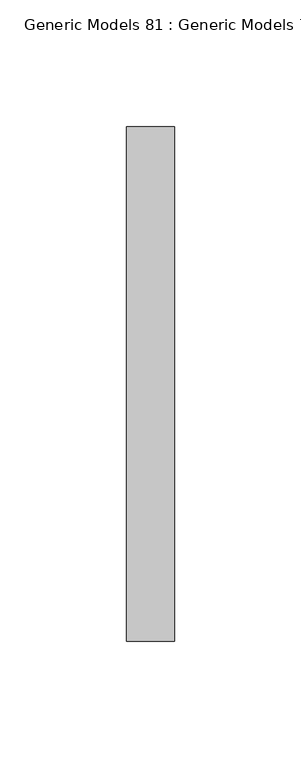
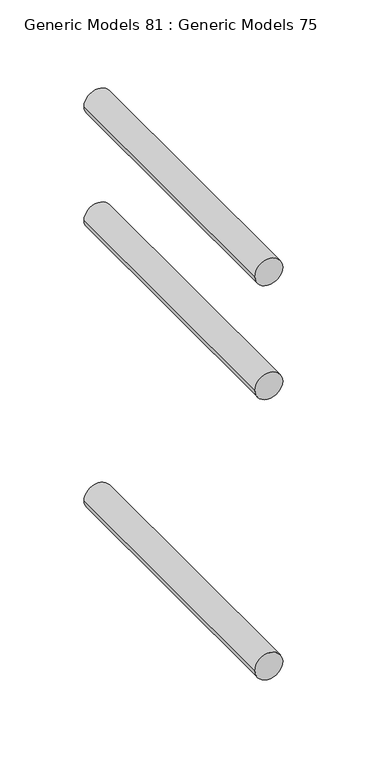
"""IFC4 building model written with IfcOpenShell, lengths in millimetres: proxy geometry, Generic Models 81 : Generic Models 75."""

import ifcopenshell
import ifcopenshell.guid

model = None  # the IFC model being written
_history = None  # IfcOwnerHistory: only IFC2X3 demands one
_inside = {}  # id of a spatial element -> (the spatial element, [elements in it])
_under = {}  # id of a project, library or spatial element -> (it, [spatial elements below it])
_declared = {}  # id of a project -> (the project, [libraries it declares])
_typed = {}  # id of a type object -> (the type object, [elements of that type])
_made_of = {}  # id of a material, layer set ... -> (it, [elements and type objects made of it])


def new_model(schema):
    """Start an empty IFC model of exactly this schema.

    Asked for "IFC4X3", IfcOpenShell would pick the latest addendum, in which some entities
    have other attributes; the version numbers below select the first issue.
    IFC2X3 requires an IfcOwnerHistory on every rooted entity: one is made here for all.
    """
    global model, _history
    if schema == "IFC4X3":
        model = ifcopenshell.file(schema_version=(4, 3, 0, 0))
    else:
        model = ifcopenshell.file(schema=schema)
    _inside.clear()
    _under.clear()
    _declared.clear()
    _typed.clear()
    _made_of.clear()
    _history = None
    if model.schema == "IFC2X3":
        org = make("IfcOrganization", Name="unknown")
        user = make(
            "IfcPersonAndOrganization",
            ThePerson=make("IfcPerson", FamilyName="unknown"),
            TheOrganization=org,
        )
        app = make(
            "IfcApplication",
            ApplicationDeveloper=org,
            Version="unknown",
            ApplicationFullName="unknown",
            ApplicationIdentifier="unknown",
        )
        _history = make(
            "IfcOwnerHistory",
            OwningUser=user,
            OwningApplication=app,
            ChangeAction="ADDED",
            CreationDate=0,
        )
    return model


def make(cls, **values):
    """One entity of the class cls with the attributes given. An attribute that is None is left unset."""
    return model.create_entity(
        cls, **{name: value for name, value in values.items() if value is not None}
    )


def rooted(cls, **values):
    """An entity with a GlobalId (a new one), such as an element, a storey or a relation."""
    return make(cls, GlobalId=ifcopenshell.guid.new(), OwnerHistory=_history, **values)


def si_unit(unit_type, name, prefix=None):
    """IfcSIUnit, for example si_unit("LENGTHUNIT", "METRE", prefix="MILLI")."""
    return make("IfcSIUnit", UnitType=unit_type, Prefix=prefix, Name=name)


def assignment(units):
    """IfcUnitAssignment: the units of a project."""
    return None if units is None else make("IfcUnitAssignment", Units=units)


def point(xyz):
    """IfcCartesianPoint."""
    return None if xyz is None else make("IfcCartesianPoint", Coordinates=xyz)


def direction(xyz):
    """IfcDirection."""
    return None if xyz is None else make("IfcDirection", DirectionRatios=xyz)


def frame(location, z_axis=None, x_axis=None):
    """IfcAxis2Placement3D, a coordinate frame: its origin and axes. An axis left out is left unset."""
    return make(
        "IfcAxis2Placement3D",
        Location=point(location),
        Axis=direction(z_axis),
        RefDirection=direction(x_axis),
    )


def frame_2d(location, x_axis=None):
    """IfcAxis2Placement2D, a coordinate frame in the plane: its origin and x axis."""
    return make(
        "IfcAxis2Placement2D", Location=point(location), RefDirection=direction(x_axis)
    )


def origin():
    """The frame at (0, 0, 0) with its axes left unset."""
    return frame((0.0, 0.0, 0.0))


def place(relative_to, where):
    """IfcLocalPlacement: puts the frame where relative to a parent placement (None: the world)."""
    return make(
        "IfcLocalPlacement", PlacementRelTo=relative_to, RelativePlacement=where
    )


def context(
    kind, dimensions, precision=None, world=None, true_north=None, identifier=None
):
    """IfcGeometricRepresentationContext, for example the 3D "Model" context."""
    return make(
        "IfcGeometricRepresentationContext",
        ContextIdentifier=identifier,
        ContextType=kind,
        CoordinateSpaceDimension=dimensions,
        Precision=precision,
        WorldCoordinateSystem=world,
        TrueNorth=true_north,
    )


def project(units=None, contexts=None):
    """IfcProject with its units and contexts."""
    return rooted(
        "IfcProject",
        Name="project",
        RepresentationContexts=contexts,
        UnitsInContext=assignment(units),
    )


def spatial(cls, under=None, at=None, **own):
    """A site, building, storey or space (cls), placed at a placement, below another one or the project."""
    s = rooted(cls, ObjectPlacement=at, **own)
    if under is not None:
        _under.setdefault(under.id(), (under, []))[1].append(s)
    return s


def circle_curve(where, radius):
    """IfcCircle in the frame where."""
    return make("IfcCircle", Position=where, Radius=radius)


def trimmed(basis, trim1, trim2, sense, master):
    """IfcTrimmedCurve: the piece of a basis curve between two trims."""
    return make(
        "IfcTrimmedCurve",
        BasisCurve=basis,
        Trim1=trim1,
        Trim2=trim2,
        SenseAgreement=sense,
        MasterRepresentation=master,
    )


def segment(curve, same_sense, transition):
    """IfcCompositeCurveSegment."""
    return make(
        "IfcCompositeCurveSegment",
        Transition=transition,
        SameSense=same_sense,
        ParentCurve=curve,
    )


def composite_curve(segments, self_intersect=None):
    """IfcCompositeCurve: segments joined end to end."""
    return make("IfcCompositeCurve", Segments=segments, SelfIntersect=self_intersect)


def outline(outer, holes=None, kind="AREA"):
    """IfcArbitraryClosedProfileDef: a profile drawn as a closed curve; with holes, ...WithVoids."""
    if holes is None:
        return make("IfcArbitraryClosedProfileDef", ProfileType=kind, OuterCurve=outer)
    return make(
        "IfcArbitraryProfileDefWithVoids",
        ProfileType=kind,
        OuterCurve=outer,
        InnerCurves=holes,
    )


def extrude(swept, where, along, depth):
    """IfcExtrudedAreaSolid: the profile swept, set in the frame where, extruded along a direction by depth."""
    return make(
        "IfcExtrudedAreaSolid",
        SweptArea=swept,
        Position=where,
        ExtrudedDirection=direction(along),
        Depth=depth,
    )


def shape(context_of_items, identifier, shape_type, items):
    """IfcShapeRepresentation: the items that make up one representation, for example the "Body"."""
    return make(
        "IfcShapeRepresentation",
        ContextOfItems=context_of_items,
        RepresentationIdentifier=identifier,
        RepresentationType=shape_type,
        Items=items,
    )


def source(mapping_origin, context_of_items, identifier, shape_type, items):
    """IfcRepresentationMap: a shape defined once, which mapped items show again and again."""
    return make(
        "IfcRepresentationMap",
        MappingOrigin=mapping_origin,
        MappedRepresentation=shape(context_of_items, identifier, shape_type, items),
    )


def transform(
    local_origin,
    x_axis=None,
    y_axis=None,
    z_axis=None,
    scale=None,
    scale2=None,
    scale3=None,
    uniform=True,
):
    """IfcCartesianTransformationOperator3D, or its non-uniform kind. x_axis, y_axis, z_axis: its Axis1, 2, 3."""
    if uniform:
        return make(
            "IfcCartesianTransformationOperator3D",
            Axis1=direction(x_axis),
            Axis2=direction(y_axis),
            LocalOrigin=point(local_origin),
            Scale=scale,
            Axis3=direction(z_axis),
        )
    return make(
        "IfcCartesianTransformationOperator3DnonUniform",
        Axis1=direction(x_axis),
        Axis2=direction(y_axis),
        LocalOrigin=point(local_origin),
        Scale=scale,
        Axis3=direction(z_axis),
        Scale2=scale2,
        Scale3=scale3,
    )


def mapped(mapping_source, mapping_target):
    """IfcMappedItem: shows the shape of a source again, moved by a transform."""
    return make(
        "IfcMappedItem", MappingSource=mapping_source, MappingTarget=mapping_target
    )


def made_of(thing, what):
    """Note that an element or type object is made of a material, layer set ...; save() writes the relation."""
    if what is not None:
        _made_of.setdefault(what.id(), (what, []))[1].append(thing)
    return thing


def element(
    cls,
    number,
    at=None,
    inside=None,
    cuts=None,
    type_object=None,
    material=None,
    context=None,
    identifier="Body",
    shape_type=None,
    held_by="IfcProductDefinitionShape",
    body=None,
    shapes=None,
    **own,
):
    """One element of the class cls, such as IfcWall. Its Tag is "e" and its number.

    at: its placement. inside: the storey or other place that contains it. cuts: it is an
    opening in that element (IfcRelVoidsElement). A single representation is given by context,
    identifier, shape_type and body (its items); several are given by shapes. held_by: the class
    of the entity that holds the representations. save() writes the other relations.
    """
    e = rooted(cls, Tag="e%d" % number, ObjectPlacement=at, **own)
    if body is not None:
        shapes = [shape(context, identifier, shape_type, body)]
    if shapes is not None:
        e.Representation = make(held_by, Representations=shapes)
    if inside is not None:
        _inside.setdefault(inside.id(), (inside, []))[1].append(e)
    if cuts is not None:
        rooted(
            "IfcRelVoidsElement", RelatingBuildingElement=cuts, RelatedOpeningElement=e
        )
    if type_object is not None:
        _typed.setdefault(type_object.id(), (type_object, []))[1].append(e)
    return made_of(e, material)


def aggregate(whole, parts):
    """IfcRelAggregates: a whole, such as a stair, and the parts it consists of."""
    return rooted("IfcRelAggregates", RelatingObject=whole, RelatedObjects=parts)


def save(model, path):
    """Write the relations noted so far, then the file.

    IfcRelAggregates (storeys below a building ...), IfcRelContainedInSpatialStructure (elements
    in a storey), IfcRelDefinesByType, IfcRelAssociatesMaterial and IfcRelDeclares: one each for
    every whole, place, type object, material and project.
    """
    for whole, parts in _under.values():
        aggregate(whole, parts)
    for where, things in _inside.values():
        rooted(
            "IfcRelContainedInSpatialStructure",
            RelatedElements=things,
            RelatingStructure=where,
        )
    for kind, things in _typed.values():
        rooted("IfcRelDefinesByType", RelatedObjects=things, RelatingType=kind)
    for what, things in _made_of.values():
        rooted("IfcRelAssociatesMaterial", RelatedObjects=things, RelatingMaterial=what)
    for by, libraries in _declared.values():
        rooted("IfcRelDeclares", RelatingContext=by, RelatedDefinitions=libraries)
    model.write(path)


def generic_models_81_generic_models_75_cf51a0b5(model_context):
    return source(origin(), model_context, "Body", "SweptSolid", [
        extrude(outline(composite_curve([segment(trimmed(circle_curve(frame_2d((271722.85, 31975.4096032)), 9.525), [point((271722.85, 31965.8846032))], [point((271722.85, 31984.9346032))], False, "CARTESIAN"), True, "CONTINUOUS"), segment(trimmed(circle_curve(frame_2d((271722.85, 31975.4096032)), 9.525), [point((271722.85, 31984.9346032))], [point((271722.85, 31965.8846032))], False, "CARTESIAN"), True, "CONTINUOUS")], self_intersect=False)), frame((0.0, 35188.2207942, 0.0), z_axis=(0.0, 1.0, 0.0), x_axis=(0.0, 0.0, 1.0)), (0.0, 0.0, 1.0), 203.2),
        extrude(outline(composite_curve([segment(trimmed(circle_curve(frame_2d((271437.1, 31975.4096032)), 9.525), [point((271437.1, 31965.8846032))], [point((271437.1, 31984.9346032))], False, "CARTESIAN"), True, "CONTINUOUS"), segment(trimmed(circle_curve(frame_2d((271437.1, 31975.4096032)), 9.525), [point((271437.1, 31984.9346032))], [point((271437.1, 31965.8846032))], False, "CARTESIAN"), True, "CONTINUOUS")], self_intersect=False)), frame((0.0, 35188.2207942, 0.0), z_axis=(0.0, 1.0, 0.0), x_axis=(0.0, 0.0, 1.0)), (0.0, 0.0, 1.0), 203.2),
        extrude(outline(composite_curve([segment(trimmed(circle_curve(frame_2d((271640.3, 31975.4096032)), 9.525), [point((271640.3, 31965.8846032))], [point((271640.3, 31984.9346032))], False, "CARTESIAN"), True, "CONTINUOUS"), segment(trimmed(circle_curve(frame_2d((271640.3, 31975.4096032)), 9.525), [point((271640.3, 31984.9346032))], [point((271640.3, 31965.8846032))], False, "CARTESIAN"), True, "CONTINUOUS")], self_intersect=False)), frame((0.0, 35188.2207942, 0.0), z_axis=(0.0, 1.0, 0.0), x_axis=(0.0, 0.0, 1.0)), (0.0, 0.0, 1.0), 203.2),
    ])


if __name__ == "__main__":
    model = new_model("IFC4")
    model_context = context("Model", 3, world=origin())
    ifc_project = project(units=[si_unit("LENGTHUNIT", "METRE", prefix="MILLI")], contexts=[model_context])
    site = spatial("IfcSite", under=ifc_project)
    building = spatial("IfcBuilding", under=site)
    placement = place(None, origin())
    generic_models_81_generic_models_75_shape = generic_models_81_generic_models_75_cf51a0b5(model_context)
    element("IfcBuildingElementProxy", 1, Name="Generic Models 81 : Generic Models 75", ObjectType="Generic Models 81 : Generic Models 75", at=placement, inside=building, context=model_context, shape_type="MappedRepresentation", body=[
        mapped(generic_models_81_generic_models_75_shape, transform((0.0, 0.0, 0.0), x_axis=(1.0, 0.0, 0.0), y_axis=(0.0, 1.0, 0.0), z_axis=(0.0, 0.0, 1.0))),
    ])
    save(model, "model.ifc")
